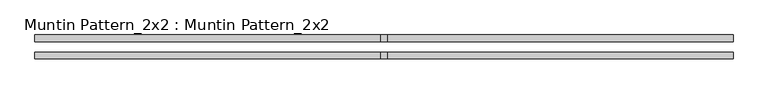
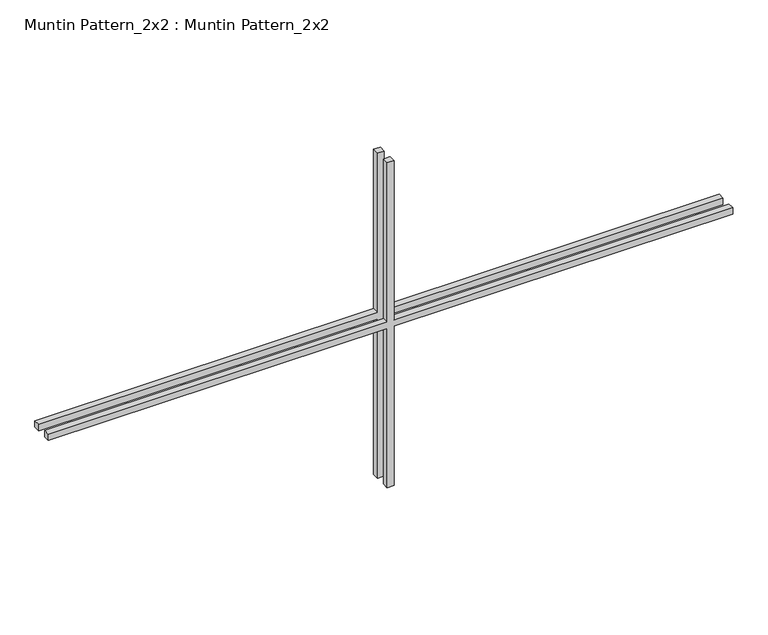
"""IFC4 building model written with IfcOpenShell, lengths in millimetres: proxy geometry, Muntin Pattern_2x2 : Muntin Pattern_2x2."""

from ifc_helpers import new_model, si_unit, frame, origin, place, context, project, spatial, polyline, outline, extrude, source, transform, mapped, element, save


def muntin_pattern_2x2_muntin_pattern_2x2_600a2e00(model_context):
    return source(origin(), model_context, "Body", "SweptSolid", [
        extrude(outline(polyline([(331.7875, -6.35), (331.7875, -647.7), (319.0875, -647.7), (319.0875, -6.35), (0.0, -6.35), (0.0, 6.35), (319.0875, 6.35), (319.0875, 647.7), (331.7875, 647.7), (331.7875, 6.35), (650.875, 6.35), (650.875, -6.35), (331.7875, -6.35)])), frame((0.0, -22.225, 0.0), z_axis=(0.0, 1.0, 0.0), x_axis=(0.0, 0.0, 1.0)), (0.0, 0.0, 1.0), 12.7),
        extrude(outline(polyline([(331.7875, -6.35), (331.7875, -647.7), (319.0875, -647.7), (319.0875, -6.35), (0.0, -6.35), (0.0, 6.35), (319.0875, 6.35), (319.0875, 647.7), (331.7875, 647.7), (331.7875, 6.35), (650.875, 6.35), (650.875, -6.35), (331.7875, -6.35)])), frame((0.0, 9.525, 0.0), z_axis=(0.0, 1.0, 0.0), x_axis=(0.0, 0.0, 1.0)), (0.0, 0.0, 1.0), 12.7),
    ])


if __name__ == "__main__":
    model = new_model("IFC4")
    model_context = context("Model", 3, world=origin())
    ifc_project = project(units=[si_unit("LENGTHUNIT", "METRE", prefix="MILLI")], contexts=[model_context])
    site = spatial("IfcSite", under=ifc_project)
    building = spatial("IfcBuilding", under=site)
    placement = place(None, origin())
    muntin_pattern_2x2_muntin_pattern_2x2_shape = muntin_pattern_2x2_muntin_pattern_2x2_600a2e00(model_context)
    element("IfcBuildingElementProxy", 1, Name="Muntin Pattern_2x2 : Muntin Pattern_2x2", ObjectType="Muntin Pattern_2x2 : Muntin Pattern_2x2", at=placement, inside=building, context=model_context, shape_type="MappedRepresentation", body=[
        mapped(muntin_pattern_2x2_muntin_pattern_2x2_shape, transform((0.0, 0.0, 0.0), x_axis=(1.0, 0.0, 0.0), y_axis=(0.0, 1.0, 0.0), z_axis=(0.0, 0.0, 1.0))),
    ])
    save(model, "model.ifc")

# Revit data of these elements
# Type "Muntin Pattern_2x2 : Muntin Pattern_2x2"
#   Width [instance default] = 4' - 0"
#   Thickness = 0' - 0 1/2"
#   Height [instance default] = 4' - 0"
#   Distance = 0' - 0 3/4"
#   Interior Material [instance default] = none
#   Exterior Material [instance default] = none
# Element 1 (IfcBuildingElementProxy, "Muntin Pattern_2x2 : Muntin Pattern_2x2")
#   Width = 4' - 3"
#   Height = 2' - 1 5/8"
#   Interior Material = Wood - Stained
#   Exterior Material = Clad - White
#   Materials on its faces: "Clad - White", "Wood - Stained"
# Materials
#   "Clad - White": class "Wood", colour RGB 242 242 238, transparency 0, Cost = 0
#   "Wood - Stained": class "Wood", colour RGB 224 178 126, transparency 0, Cost = 0
